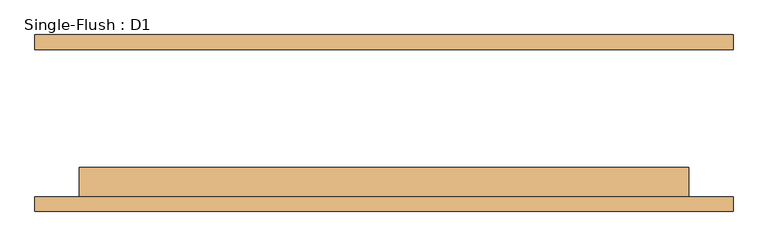
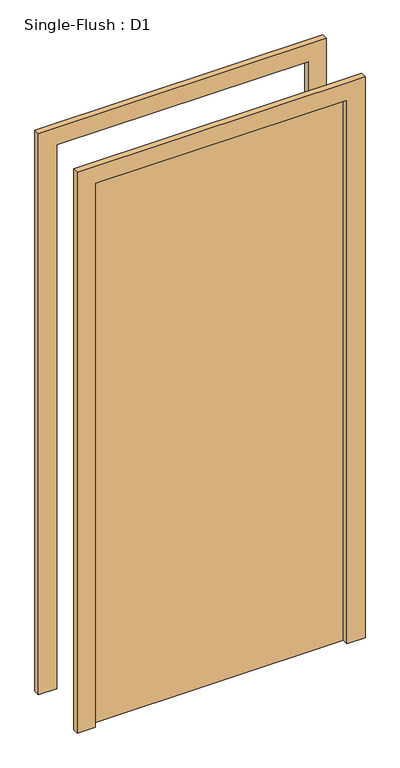
"""IFC4 building model written with IfcOpenShell, lengths in millimetres: door geometry, Single-Flush : D1."""

import ifcopenshell
import ifcopenshell.guid

model = None  # the IFC model being written
_history = None  # IfcOwnerHistory: only IFC2X3 demands one
_inside = {}  # id of a spatial element -> (the spatial element, [elements in it])
_under = {}  # id of a project, library or spatial element -> (it, [spatial elements below it])
_declared = {}  # id of a project -> (the project, [libraries it declares])
_typed = {}  # id of a type object -> (the type object, [elements of that type])
_made_of = {}  # id of a material, layer set ... -> (it, [elements and type objects made of it])


def new_model(schema):
    """Start an empty IFC model of exactly this schema.

    Asked for "IFC4X3", IfcOpenShell would pick the latest addendum, in which some entities
    have other attributes; the version numbers below select the first issue.
    IFC2X3 requires an IfcOwnerHistory on every rooted entity: one is made here for all.
    """
    global model, _history
    if schema == "IFC4X3":
        model = ifcopenshell.file(schema_version=(4, 3, 0, 0))
    else:
        model = ifcopenshell.file(schema=schema)
    _inside.clear()
    _under.clear()
    _declared.clear()
    _typed.clear()
    _made_of.clear()
    _history = None
    if model.schema == "IFC2X3":
        org = make("IfcOrganization", Name="unknown")
        user = make(
            "IfcPersonAndOrganization",
            ThePerson=make("IfcPerson", FamilyName="unknown"),
            TheOrganization=org,
        )
        app = make(
            "IfcApplication",
            ApplicationDeveloper=org,
            Version="unknown",
            ApplicationFullName="unknown",
            ApplicationIdentifier="unknown",
        )
        _history = make(
            "IfcOwnerHistory",
            OwningUser=user,
            OwningApplication=app,
            ChangeAction="ADDED",
            CreationDate=0,
        )
    return model


def make(cls, **values):
    """One entity of the class cls with the attributes given. An attribute that is None is left unset."""
    return model.create_entity(
        cls, **{name: value for name, value in values.items() if value is not None}
    )


def rooted(cls, **values):
    """An entity with a GlobalId (a new one), such as an element, a storey or a relation."""
    return make(cls, GlobalId=ifcopenshell.guid.new(), OwnerHistory=_history, **values)


def si_unit(unit_type, name, prefix=None):
    """IfcSIUnit, for example si_unit("LENGTHUNIT", "METRE", prefix="MILLI")."""
    return make("IfcSIUnit", UnitType=unit_type, Prefix=prefix, Name=name)


def assignment(units):
    """IfcUnitAssignment: the units of a project."""
    return None if units is None else make("IfcUnitAssignment", Units=units)


def point(xyz):
    """IfcCartesianPoint."""
    return None if xyz is None else make("IfcCartesianPoint", Coordinates=xyz)


def direction(xyz):
    """IfcDirection."""
    return None if xyz is None else make("IfcDirection", DirectionRatios=xyz)


def frame(location, z_axis=None, x_axis=None):
    """IfcAxis2Placement3D, a coordinate frame: its origin and axes. An axis left out is left unset."""
    return make(
        "IfcAxis2Placement3D",
        Location=point(location),
        Axis=direction(z_axis),
        RefDirection=direction(x_axis),
    )


def origin():
    """The frame at (0, 0, 0) with its axes left unset."""
    return frame((0.0, 0.0, 0.0))


def origin_with_axes():
    """The frame at (0, 0, 0) with the z axis (0, 0, 1) and the x axis (1, 0, 0) written out."""
    return frame((0.0, 0.0, 0.0), z_axis=(0.0, 0.0, 1.0), x_axis=(1.0, 0.0, 0.0))


def place(relative_to, where):
    """IfcLocalPlacement: puts the frame where relative to a parent placement (None: the world)."""
    return make(
        "IfcLocalPlacement", PlacementRelTo=relative_to, RelativePlacement=where
    )


def context(
    kind, dimensions, precision=None, world=None, true_north=None, identifier=None
):
    """IfcGeometricRepresentationContext, for example the 3D "Model" context."""
    return make(
        "IfcGeometricRepresentationContext",
        ContextIdentifier=identifier,
        ContextType=kind,
        CoordinateSpaceDimension=dimensions,
        Precision=precision,
        WorldCoordinateSystem=world,
        TrueNorth=true_north,
    )


def project(units=None, contexts=None):
    """IfcProject with its units and contexts."""
    return rooted(
        "IfcProject",
        Name="project",
        RepresentationContexts=contexts,
        UnitsInContext=assignment(units),
    )


def spatial(cls, under=None, at=None, **own):
    """A site, building, storey or space (cls), placed at a placement, below another one or the project."""
    s = rooted(cls, ObjectPlacement=at, **own)
    if under is not None:
        _under.setdefault(under.id(), (under, []))[1].append(s)
    return s


def polyline(points):
    """IfcPolyline through the points."""
    return make("IfcPolyline", Points=[point(p) for p in points])


def outline(outer, holes=None, kind="AREA"):
    """IfcArbitraryClosedProfileDef: a profile drawn as a closed curve; with holes, ...WithVoids."""
    if holes is None:
        return make("IfcArbitraryClosedProfileDef", ProfileType=kind, OuterCurve=outer)
    return make(
        "IfcArbitraryProfileDefWithVoids",
        ProfileType=kind,
        OuterCurve=outer,
        InnerCurves=holes,
    )


def extrude(swept, where, along, depth):
    """IfcExtrudedAreaSolid: the profile swept, set in the frame where, extruded along a direction by depth."""
    return make(
        "IfcExtrudedAreaSolid",
        SweptArea=swept,
        Position=where,
        ExtrudedDirection=direction(along),
        Depth=depth,
    )


def shape(context_of_items, identifier, shape_type, items):
    """IfcShapeRepresentation: the items that make up one representation, for example the "Body"."""
    return make(
        "IfcShapeRepresentation",
        ContextOfItems=context_of_items,
        RepresentationIdentifier=identifier,
        RepresentationType=shape_type,
        Items=items,
    )


def source(mapping_origin, context_of_items, identifier, shape_type, items):
    """IfcRepresentationMap: a shape defined once, which mapped items show again and again."""
    return make(
        "IfcRepresentationMap",
        MappingOrigin=mapping_origin,
        MappedRepresentation=shape(context_of_items, identifier, shape_type, items),
    )


def transform(
    local_origin,
    x_axis=None,
    y_axis=None,
    z_axis=None,
    scale=None,
    scale2=None,
    scale3=None,
    uniform=True,
):
    """IfcCartesianTransformationOperator3D, or its non-uniform kind. x_axis, y_axis, z_axis: its Axis1, 2, 3."""
    if uniform:
        return make(
            "IfcCartesianTransformationOperator3D",
            Axis1=direction(x_axis),
            Axis2=direction(y_axis),
            LocalOrigin=point(local_origin),
            Scale=scale,
            Axis3=direction(z_axis),
        )
    return make(
        "IfcCartesianTransformationOperator3DnonUniform",
        Axis1=direction(x_axis),
        Axis2=direction(y_axis),
        LocalOrigin=point(local_origin),
        Scale=scale,
        Axis3=direction(z_axis),
        Scale2=scale2,
        Scale3=scale3,
    )


def mapped(mapping_source, mapping_target):
    """IfcMappedItem: shows the shape of a source again, moved by a transform."""
    return make(
        "IfcMappedItem", MappingSource=mapping_source, MappingTarget=mapping_target
    )


def made_of(thing, what):
    """Note that an element or type object is made of a material, layer set ...; save() writes the relation."""
    if what is not None:
        _made_of.setdefault(what.id(), (what, []))[1].append(thing)
    return thing


def element(
    cls,
    number,
    at=None,
    inside=None,
    cuts=None,
    type_object=None,
    material=None,
    context=None,
    identifier="Body",
    shape_type=None,
    held_by="IfcProductDefinitionShape",
    body=None,
    shapes=None,
    **own,
):
    """One element of the class cls, such as IfcWall. Its Tag is "e" and its number.

    at: its placement. inside: the storey or other place that contains it. cuts: it is an
    opening in that element (IfcRelVoidsElement). A single representation is given by context,
    identifier, shape_type and body (its items); several are given by shapes. held_by: the class
    of the entity that holds the representations. save() writes the other relations.
    """
    e = rooted(cls, Tag="e%d" % number, ObjectPlacement=at, **own)
    if body is not None:
        shapes = [shape(context, identifier, shape_type, body)]
    if shapes is not None:
        e.Representation = make(held_by, Representations=shapes)
    if inside is not None:
        _inside.setdefault(inside.id(), (inside, []))[1].append(e)
    if cuts is not None:
        rooted(
            "IfcRelVoidsElement", RelatingBuildingElement=cuts, RelatedOpeningElement=e
        )
    if type_object is not None:
        _typed.setdefault(type_object.id(), (type_object, []))[1].append(e)
    return made_of(e, material)


def aggregate(whole, parts):
    """IfcRelAggregates: a whole, such as a stair, and the parts it consists of."""
    return rooted("IfcRelAggregates", RelatingObject=whole, RelatedObjects=parts)


def save(model, path):
    """Write the relations noted so far, then the file.

    IfcRelAggregates (storeys below a building ...), IfcRelContainedInSpatialStructure (elements
    in a storey), IfcRelDefinesByType, IfcRelAssociatesMaterial and IfcRelDeclares: one each for
    every whole, place, type object, material and project.
    """
    for whole, parts in _under.values():
        aggregate(whole, parts)
    for where, things in _inside.values():
        rooted(
            "IfcRelContainedInSpatialStructure",
            RelatedElements=things,
            RelatingStructure=where,
        )
    for kind, things in _typed.values():
        rooted("IfcRelDefinesByType", RelatedObjects=things, RelatingType=kind)
    for what, things in _made_of.values():
        rooted("IfcRelAssociatesMaterial", RelatedObjects=things, RelatingMaterial=what)
    for by, libraries in _declared.values():
        rooted("IfcRelDeclares", RelatingContext=by, RelatedDefinitions=libraries)
    model.write(path)


def single_flush_d1_c0f18f60(model_context):
    return source(origin(), model_context, "Body", "SweptSolid", [
        extrude(outline(polyline([(2476.2, -601.2), (0.0, -601.2), (0.0, -525.0), (2400.0, -525.0), (2400.0, 525.0), (0.0, 525.0), (0.0, 601.2), (2476.2, 601.2), (2476.2, -601.2)])), frame((0.0, -152.4, 0.0), z_axis=(0.0, 1.0, 0.0), x_axis=(0.0, 0.0, 1.0)), (0.0, 0.0, 1.0), 25.4),
        extrude(outline(polyline([(2476.2, 601.2), (2476.2, -601.2), (0.0, -601.2), (0.0, -525.0), (2400.0, -525.0), (2400.0, 525.0), (0.0, 525.0), (0.0, 601.2), (2476.2, 601.2)])), frame((0.0, 127.0, 0.0), z_axis=(0.0, 1.0, 0.0), x_axis=(0.0, 0.0, 1.0)), (0.0, 0.0, 1.0), 25.4),
        extrude(outline(polyline([(525.0, -76.2), (525.0, -127.0), (-525.0, -127.0), (-525.0, -76.2), (525.0, -76.2)])), origin_with_axes(), (0.0, 0.0, 1.0), 2400.0),
    ])


if __name__ == "__main__":
    model = new_model("IFC4")
    model_context = context("Model", 3, world=origin())
    ifc_project = project(units=[si_unit("LENGTHUNIT", "METRE", prefix="MILLI")], contexts=[model_context])
    site = spatial("IfcSite", under=ifc_project)
    building = spatial("IfcBuilding", under=site)
    placement = place(None, origin())
    single_flush_d1_shape = single_flush_d1_c0f18f60(model_context)
    element("IfcDoor", 1, ObjectType="Single-Flush : D1", at=placement, inside=building, context=model_context, shape_type="MappedRepresentation", body=[
        mapped(single_flush_d1_shape, transform((0.0, 0.0, 0.0), x_axis=(1.0, 0.0, 0.0), y_axis=(0.0, 1.0, 0.0), z_axis=(0.0, 0.0, 1.0))),
    ])
    save(model, "model.ifc")

# Revit data of these elements
# Type "Single-Flush : D1"
#   Type Mark = "D1"
#   Construction Type Id = "MDOOR"
#   Assembly Code = "C1020"
#   Analytic Construction = "Metal"
#   Thickness = 50.8 mm
#   Heat Transfer Coefficient (U) = 3.7021 W/(m²·K)
#   Height = 2400 mm
#   Trim Projection Ext = 25.4 mm
#   Trim Projection Int = 25.4 mm
#   Trim Width = 76.2 mm
#   Width = 1050 mm
#   Door Material = Door - Panel
#   Frame Material = Door - Frame
#   Visual Light Transmittance = 0
#   Solar Heat Gain Coefficient = 0
#   Function = (empty or 0)
#   Wall Closure = (empty or 0)
# Element 1 (IfcDoor, "Single-Flush : D1")
#   Materials on its faces: "Door - Frame", "Door - Panel"
# Materials
#   "Door - Panel": class "Wood", colour RGB 210 159 95, transparency 0
#   "Door - Frame": class "Miscellaneous", colour RGB 118 70 51, transparency 0
